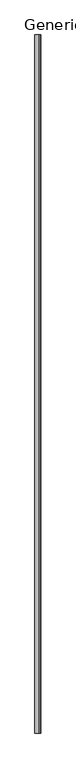
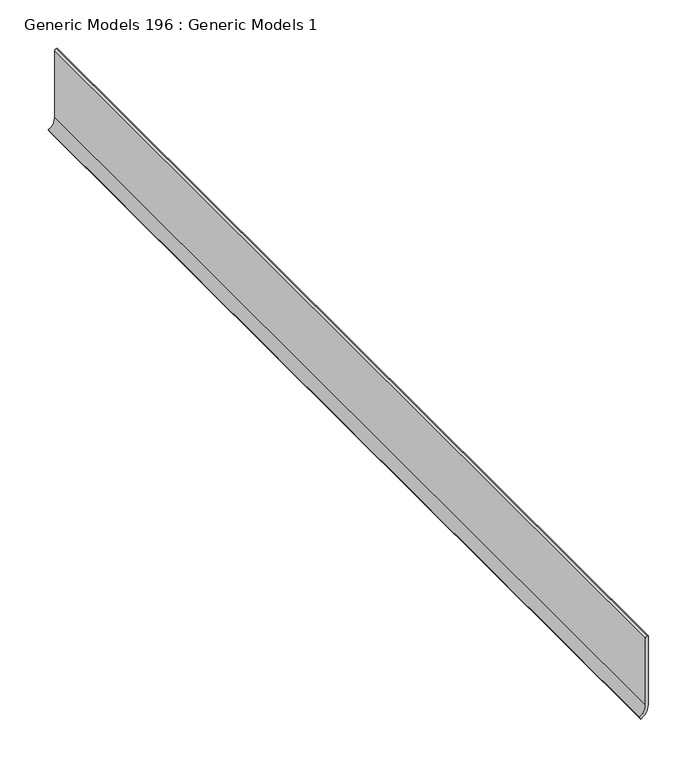
"""IFC4 building model written with IfcOpenShell, lengths in millimetres: proxy geometry, Generic Models 196 : Generic Models 1."""

from ifc_helpers import new_model, si_unit, point, frame, frame_2d, origin, place, context, project, spatial, polyline, circle_curve, trimmed, segment, composite_curve, outline, extrude, source, transform, mapped, element, save


def generic_models_196_generic_models_1_c5b7b2a8(model_context):
    return source(origin(), model_context, "Body", "SweptSolid", [
        extrude(outline(composite_curve([segment(polyline([(101.6, 49676.05), (101.6, 49674.9618018)]), True, "CONTINUOUS"), segment(trimmed(circle_curve(frame_2d((99.5131982, 49674.9618018)), 2.0868018), [point((101.6, 49674.9618018))], [point((99.5131982, 49672.875))], False, "CARTESIAN"), True, "CONTINUOUS"), segment(polyline([(99.5131982, 49672.875), (15.4496307, 49672.875)]), True, "CONTINUOUS"), segment(trimmed(circle_curve(frame_2d((15.4496307, 49658.2103032)), 14.6646968), [point((15.4496307, 49672.875))], [point((2.7496307, 49665.5426516))], True, "CARTESIAN"), True, "CONTINUOUS"), segment(polyline([(2.7496307, 49665.5426516), (0.0, 49667.1301516)]), True, "CONTINUOUS"), segment(trimmed(circle_curve(frame_2d((15.4496307, 49658.2103032)), 17.8396968), [point((0.0, 49667.1301516))], [point((15.4496307, 49676.05))], False, "CARTESIAN"), True, "CONTINUOUS"), segment(polyline([(15.4496307, 49676.05), (101.6, 49676.05)]), True, "CONTINUOUS")], self_intersect=False)), frame((0.0, 0.0, 0.0), z_axis=(0.0, 1.0, 0.0), x_axis=(0.0, 0.0, 1.0)), (0.0, 0.0, 1.0), 1219.2),
    ])


if __name__ == "__main__":
    model = new_model("IFC4")
    model_context = context("Model", 3, world=origin())
    ifc_project = project(units=[si_unit("LENGTHUNIT", "METRE", prefix="MILLI")], contexts=[model_context])
    site = spatial("IfcSite", under=ifc_project)
    building = spatial("IfcBuilding", under=site)
    placement = place(None, origin())
    generic_models_196_generic_models_1_shape = generic_models_196_generic_models_1_c5b7b2a8(model_context)
    element("IfcBuildingElementProxy", 1, Name="Generic Models 196 : Generic Models 1", ObjectType="Generic Models 196 : Generic Models 1", at=placement, inside=building, context=model_context, shape_type="MappedRepresentation", body=[
        mapped(generic_models_196_generic_models_1_shape, transform((0.0, 0.0, 0.0), x_axis=(1.0, 0.0, 0.0), y_axis=(0.0, 1.0, 0.0), z_axis=(0.0, 0.0, 1.0))),
    ])
    save(model, "model.ifc")

# Revit data of these elements
# Element 1 (IfcBuildingElementProxy, "Generic Models 196 : Generic Models 1")
#   Materials on its faces: "MATCH EXISTING BASE"
# Materials
#   "MATCH EXISTING BASE": class "Generic", colour RGB 120 120 120, transparency 0, Cost = 0
